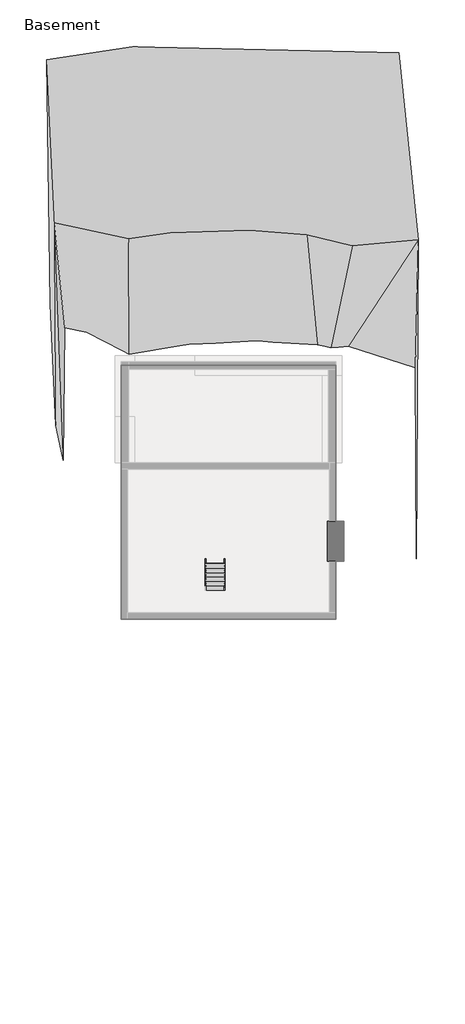
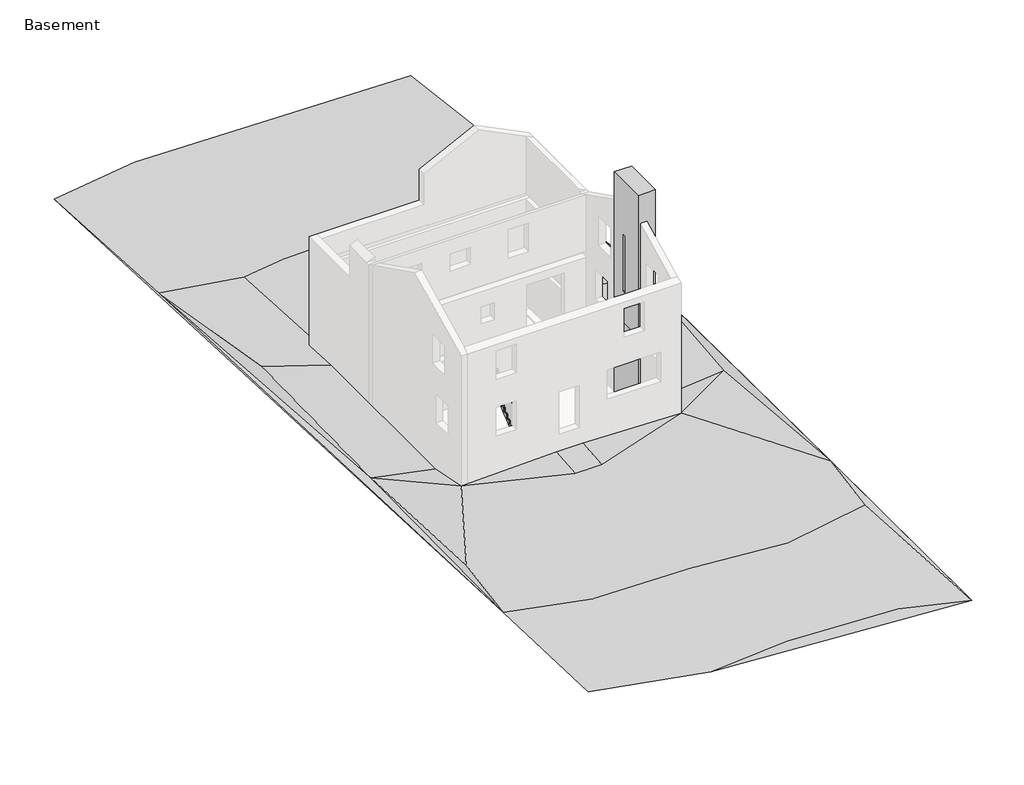
# One storey, part 2 of 2: 4 proxies, 2 members, 1 railing, 1 stair flight.
"""IFC4 building model written with IfcOpenShell, lengths in millimetres."""

import ifcopenshell
import ifcopenshell.guid

model = None  # the IFC model being written
_history = None  # IfcOwnerHistory: only IFC2X3 demands one
_inside = {}  # id of a spatial element -> (the spatial element, [elements in it])
_under = {}  # id of a project, library or spatial element -> (it, [spatial elements below it])
_declared = {}  # id of a project -> (the project, [libraries it declares])
_typed = {}  # id of a type object -> (the type object, [elements of that type])
_made_of = {}  # id of a material, layer set ... -> (it, [elements and type objects made of it])


def new_model(schema):
    """Start an empty IFC model of exactly this schema.

    Asked for "IFC4X3", IfcOpenShell would pick the latest addendum, in which some entities
    have other attributes; the version numbers below select the first issue.
    IFC2X3 requires an IfcOwnerHistory on every rooted entity: one is made here for all.
    """
    global model, _history
    if schema == "IFC4X3":
        model = ifcopenshell.file(schema_version=(4, 3, 0, 0))
    else:
        model = ifcopenshell.file(schema=schema)
    _inside.clear()
    _under.clear()
    _declared.clear()
    _typed.clear()
    _made_of.clear()
    _history = None
    if model.schema == "IFC2X3":
        org = make("IfcOrganization", Name="unknown")
        user = make(
            "IfcPersonAndOrganization",
            ThePerson=make("IfcPerson", FamilyName="unknown"),
            TheOrganization=org,
        )
        app = make(
            "IfcApplication",
            ApplicationDeveloper=org,
            Version="unknown",
            ApplicationFullName="unknown",
            ApplicationIdentifier="unknown",
        )
        _history = make(
            "IfcOwnerHistory",
            OwningUser=user,
            OwningApplication=app,
            ChangeAction="ADDED",
            CreationDate=0,
        )
    return model


def make(cls, **values):
    """One entity of the class cls with the attributes given. An attribute that is None is left unset."""
    return model.create_entity(
        cls, **{name: value for name, value in values.items() if value is not None}
    )


def rooted(cls, **values):
    """An entity with a GlobalId (a new one), such as an element, a storey or a relation."""
    return make(cls, GlobalId=ifcopenshell.guid.new(), OwnerHistory=_history, **values)


def si_unit(unit_type, name, prefix=None):
    """IfcSIUnit, for example si_unit("LENGTHUNIT", "METRE", prefix="MILLI")."""
    return make("IfcSIUnit", UnitType=unit_type, Prefix=prefix, Name=name)


def assignment(units):
    """IfcUnitAssignment: the units of a project."""
    return None if units is None else make("IfcUnitAssignment", Units=units)


def point(xyz):
    """IfcCartesianPoint."""
    return None if xyz is None else make("IfcCartesianPoint", Coordinates=xyz)


def direction(xyz):
    """IfcDirection."""
    return None if xyz is None else make("IfcDirection", DirectionRatios=xyz)


def frame(location, z_axis=None, x_axis=None):
    """IfcAxis2Placement3D, a coordinate frame: its origin and axes. An axis left out is left unset."""
    return make(
        "IfcAxis2Placement3D",
        Location=point(location),
        Axis=direction(z_axis),
        RefDirection=direction(x_axis),
    )


def origin():
    """The frame at (0, 0, 0) with its axes left unset."""
    return frame((0.0, 0.0, 0.0))


def place(relative_to, where):
    """IfcLocalPlacement: puts the frame where relative to a parent placement (None: the world)."""
    return make(
        "IfcLocalPlacement", PlacementRelTo=relative_to, RelativePlacement=where
    )


def context(
    kind, dimensions, precision=None, world=None, true_north=None, identifier=None
):
    """IfcGeometricRepresentationContext, for example the 3D "Model" context."""
    return make(
        "IfcGeometricRepresentationContext",
        ContextIdentifier=identifier,
        ContextType=kind,
        CoordinateSpaceDimension=dimensions,
        Precision=precision,
        WorldCoordinateSystem=world,
        TrueNorth=true_north,
    )


def project(units=None, contexts=None):
    """IfcProject with its units and contexts."""
    return rooted(
        "IfcProject",
        Name="project",
        RepresentationContexts=contexts,
        UnitsInContext=assignment(units),
    )


def spatial(cls, under=None, at=None, **own):
    """A site, building, storey or space (cls), placed at a placement, below another one or the project."""
    s = rooted(cls, ObjectPlacement=at, **own)
    if under is not None:
        _under.setdefault(under.id(), (under, []))[1].append(s)
    return s


def polyline(points):
    """IfcPolyline through the points."""
    return make("IfcPolyline", Points=[point(p) for p in points])


def point_list(points):
    """IfcCartesianPointList2D or 3D."""
    cls = (
        "IfcCartesianPointList2D" if len(points[0]) == 2 else "IfcCartesianPointList3D"
    )
    return make(cls, CoordList=points)


def outline(outer, holes=None, kind="AREA"):
    """IfcArbitraryClosedProfileDef: a profile drawn as a closed curve; with holes, ...WithVoids."""
    if holes is None:
        return make("IfcArbitraryClosedProfileDef", ProfileType=kind, OuterCurve=outer)
    return make(
        "IfcArbitraryProfileDefWithVoids",
        ProfileType=kind,
        OuterCurve=outer,
        InnerCurves=holes,
    )


def extrude(swept, where, along, depth):
    """IfcExtrudedAreaSolid: the profile swept, set in the frame where, extruded along a direction by depth."""
    return make(
        "IfcExtrudedAreaSolid",
        SweptArea=swept,
        Position=where,
        ExtrudedDirection=direction(along),
        Depth=depth,
    )


def faces_of(points, faces, orient=None, outer=None):
    """IfcFace entities. A face is a list of loops; a loop is a list of indices into points, from 0.

    orient and outer hold one flag for each loop. By default every Orientation is true, the
    first loop of a face is its IfcFaceOuterBound and the others are IfcFaceBound.
    """
    made = []
    for i, loops in enumerate(faces):
        bounds = []
        for j, loop in enumerate(loops):
            is_outer = j == 0 if outer is None else outer[i][j]
            bounds.append(
                make(
                    "IfcFaceOuterBound" if is_outer else "IfcFaceBound",
                    Bound=make("IfcPolyLoop", Polygon=[points[k] for k in loop]),
                    Orientation=True if orient is None else orient[i][j],
                )
            )
        made.append(make("IfcFace", Bounds=bounds))
    return made


def faceted_brep(points, faces, orient=None, outer=None, voids=None):
    """IfcFacetedBrep: a solid bounded by flat faces; with voids (closed shells), ...WithVoids."""
    shared = [point(p) for p in points]
    hull = make("IfcClosedShell", CfsFaces=faces_of(shared, faces, orient, outer))
    if voids is None:
        return make("IfcFacetedBrep", Outer=hull)
    return make(
        "IfcFacetedBrepWithVoids",
        Outer=hull,
        Voids=[
            make(cls, CfsFaces=faces_of(shared, fs, o, b)) for cls, fs, o, b in voids
        ],
    )


def triangles(points, corners, closed=None, point_numbers=None):
    """IfcTriangulatedFaceSet: each triangle names its three corners, points numbered from 1."""
    return make(
        "IfcTriangulatedFaceSet",
        Coordinates=point_list(points),
        Closed=closed,
        CoordIndex=corners,
        PnIndex=point_numbers,
    )


def shape(context_of_items, identifier, shape_type, items):
    """IfcShapeRepresentation: the items that make up one representation, for example the "Body"."""
    return make(
        "IfcShapeRepresentation",
        ContextOfItems=context_of_items,
        RepresentationIdentifier=identifier,
        RepresentationType=shape_type,
        Items=items,
    )


def source(mapping_origin, context_of_items, identifier, shape_type, items):
    """IfcRepresentationMap: a shape defined once, which mapped items show again and again."""
    return make(
        "IfcRepresentationMap",
        MappingOrigin=mapping_origin,
        MappedRepresentation=shape(context_of_items, identifier, shape_type, items),
    )


def transform(
    local_origin,
    x_axis=None,
    y_axis=None,
    z_axis=None,
    scale=None,
    scale2=None,
    scale3=None,
    uniform=True,
):
    """IfcCartesianTransformationOperator3D, or its non-uniform kind. x_axis, y_axis, z_axis: its Axis1, 2, 3."""
    if uniform:
        return make(
            "IfcCartesianTransformationOperator3D",
            Axis1=direction(x_axis),
            Axis2=direction(y_axis),
            LocalOrigin=point(local_origin),
            Scale=scale,
            Axis3=direction(z_axis),
        )
    return make(
        "IfcCartesianTransformationOperator3DnonUniform",
        Axis1=direction(x_axis),
        Axis2=direction(y_axis),
        LocalOrigin=point(local_origin),
        Scale=scale,
        Axis3=direction(z_axis),
        Scale2=scale2,
        Scale3=scale3,
    )


def mapped(mapping_source, mapping_target):
    """IfcMappedItem: shows the shape of a source again, moved by a transform."""
    return make(
        "IfcMappedItem", MappingSource=mapping_source, MappingTarget=mapping_target
    )


def made_of(thing, what):
    """Note that an element or type object is made of a material, layer set ...; save() writes the relation."""
    if what is not None:
        _made_of.setdefault(what.id(), (what, []))[1].append(thing)
    return thing


def element(
    cls,
    number,
    at=None,
    inside=None,
    cuts=None,
    type_object=None,
    material=None,
    context=None,
    identifier="Body",
    shape_type=None,
    held_by="IfcProductDefinitionShape",
    body=None,
    shapes=None,
    **own,
):
    """One element of the class cls, such as IfcWall. Its Tag is "e" and its number.

    at: its placement. inside: the storey or other place that contains it. cuts: it is an
    opening in that element (IfcRelVoidsElement). A single representation is given by context,
    identifier, shape_type and body (its items); several are given by shapes. held_by: the class
    of the entity that holds the representations. save() writes the other relations.
    """
    e = rooted(cls, Tag="e%d" % number, ObjectPlacement=at, **own)
    if body is not None:
        shapes = [shape(context, identifier, shape_type, body)]
    if shapes is not None:
        e.Representation = make(held_by, Representations=shapes)
    if inside is not None:
        _inside.setdefault(inside.id(), (inside, []))[1].append(e)
    if cuts is not None:
        rooted(
            "IfcRelVoidsElement", RelatingBuildingElement=cuts, RelatedOpeningElement=e
        )
    if type_object is not None:
        _typed.setdefault(type_object.id(), (type_object, []))[1].append(e)
    return made_of(e, material)


def aggregate(whole, parts):
    """IfcRelAggregates: a whole, such as a stair, and the parts it consists of."""
    return rooted("IfcRelAggregates", RelatingObject=whole, RelatedObjects=parts)


def save(model, path):
    """Write the relations noted so far, then the file.

    IfcRelAggregates (storeys below a building ...), IfcRelContainedInSpatialStructure (elements
    in a storey), IfcRelDefinesByType, IfcRelAssociatesMaterial and IfcRelDeclares: one each for
    every whole, place, type object, material and project.
    """
    for whole, parts in _under.values():
        aggregate(whole, parts)
    for where, things in _inside.values():
        rooted(
            "IfcRelContainedInSpatialStructure",
            RelatedElements=things,
            RelatingStructure=where,
        )
    for kind, things in _typed.values():
        rooted("IfcRelDefinesByType", RelatedObjects=things, RelatingType=kind)
    for what, things in _made_of.values():
        rooted("IfcRelAssociatesMaterial", RelatedObjects=things, RelatingMaterial=what)
    for by, libraries in _declared.values():
        rooted("IfcRelDeclares", RelatingContext=by, RelatedDefinitions=libraries)
    model.write(path)


def existing_fireplace_existing_fireplace_287aed51(model_context):
    return source(origin(), model_context, "Body", "Brep", [
        faceted_brep([(4450.2196932, 434.2888758, 8077.2), (3662.8196932, 434.2888758, 8077.2), (3662.8196932, -1445.3111242, 8077.2), (4450.2196932, -1445.3111242, 8077.2), (4450.2196932, 434.2888758, -2667.0), (4450.2196932, -1445.3111242, -2667.0), (4069.2196932, -1445.3111242, -2667.0), (3764.4196932, -1445.3111242, -2667.0), (3662.8196932, -1445.3111242, -2667.0), (3662.8196932, 434.2888758, -2667.0), (3764.4196932, 434.2888758, -2667.0), (4069.2196932, 434.2888758, -2667.0), (3662.8196932, 154.8888758, 0.0), (3662.8196932, 154.8888758, 1219.2), (3662.8196932, -1165.9111242, 1219.2), (3662.8196932, -1165.9111242, 0.0), (3662.8196932, -403.9111242, 5486.4), (3662.8196932, -403.9111242, 2743.2), (3662.8196932, -276.9111242, 2743.2), (3662.8196932, -276.9111242, 5486.4), (4145.4196932, -20.7631592, 1219.2), (4145.4196932, -990.2590891, 1219.2), (4145.4196932, -990.2590891, 0.0), (4145.4196932, -20.7631592, 0.0), (3767.2567114, -403.9111242, 5486.4), (3767.2567114, -403.9111242, 2743.2), (3767.2567114, -276.9111242, 2743.2), (3767.2567114, -276.9111242, 5486.4)], [[[0, 1, 2, 3]], [[4, 5, 6, 7, 8, 9, 10, 11]], [[1, 0, 4, 11, 10, 9]], [[2, 1, 9, 8], [12, 13, 14, 15], [16, 17, 18, 19]], [[3, 2, 8, 7, 6, 5]], [[0, 3, 5, 4]], [[14, 13, 20, 21]], [[15, 14, 21, 22]], [[21, 20, 23, 22]], [[13, 12, 23, 20]], [[12, 15, 22, 23]], [[24, 25, 17, 16]], [[26, 27, 19, 18]], [[25, 26, 18, 17]], [[25, 24, 27, 26]], [[27, 24, 16, 19]]]),
    ])


def stair_flight_b746b64e(model_context):
    return source(origin(), model_context, "Body", "SweptSolid", [
        extrude(outline(polyline([(-2791.5111242, -2476.5), (-2562.9111242, -2476.5), (-2562.9111242, -2527.3), (-2766.1111242, -2527.3), (-2766.1111242, -2520.95), (-2791.5111242, -2495.55), (-2791.5111242, -2476.5)])), frame((-2052.1803068, 0.0, 0.0), z_axis=(1.0, 0.0, 0.0), x_axis=(0.0, 1.0, 0.0)), (0.0, 0.0, 1.0), 939.8),
        extrude(outline(polyline([(-1112.3803068, -2759.7611242), (-1112.3803068, -2766.1111242), (-2052.1803068, -2766.1111242), (-2052.1803068, -2759.7611242), (-1112.3803068, -2759.7611242)])), frame((0.0, 0.0, -2667.0), z_axis=(0.0, 0.0, 1.0), x_axis=(1.0, 0.0, 0.0)), (0.0, 0.0, 1.0), 139.7),
        extrude(outline(polyline([(-1112.3803068, -2556.5611242), (-1112.3803068, -2562.9111242), (-2052.1803068, -2562.9111242), (-2052.1803068, -2556.5611242), (-1112.3803068, -2556.5611242)])), frame((0.0, 0.0, -2527.3), z_axis=(0.0, 0.0, 1.0), x_axis=(1.0, 0.0, 0.0)), (0.0, 0.0, 1.0), 190.5),
        extrude(outline(polyline([(-2588.3111242, -2286.0), (-2359.7111242, -2286.0), (-2359.7111242, -2336.8), (-2562.9111242, -2336.8), (-2562.9111242, -2330.45), (-2588.3111242, -2305.05), (-2588.3111242, -2286.0)])), frame((-2052.1803068, 0.0, 0.0), z_axis=(1.0, 0.0, 0.0), x_axis=(0.0, 1.0, 0.0)), (0.0, 0.0, 1.0), 939.8),
        extrude(outline(polyline([(-1112.3803068, -2353.3611242), (-1112.3803068, -2359.7111242), (-2052.1803068, -2359.7111242), (-2052.1803068, -2353.3611242), (-1112.3803068, -2353.3611242)])), frame((0.0, 0.0, -2336.8), z_axis=(0.0, 0.0, 1.0), x_axis=(1.0, 0.0, 0.0)), (0.0, 0.0, 1.0), 190.5),
        extrude(outline(polyline([(-2385.1111242, -2095.5), (-2156.5111242, -2095.5), (-2156.5111242, -2146.3), (-2359.7111242, -2146.3), (-2359.7111242, -2139.95), (-2385.1111242, -2114.55), (-2385.1111242, -2095.5)])), frame((-2052.1803068, 0.0, 0.0), z_axis=(1.0, 0.0, 0.0), x_axis=(0.0, 1.0, 0.0)), (0.0, 0.0, 1.0), 939.8),
        extrude(outline(polyline([(-1112.3803068, -2150.1611242), (-1112.3803068, -2156.5111242), (-2052.1803068, -2156.5111242), (-2052.1803068, -2150.1611242), (-1112.3803068, -2150.1611242)])), frame((0.0, 0.0, -2146.3), z_axis=(0.0, 0.0, 1.0), x_axis=(1.0, 0.0, 0.0)), (0.0, 0.0, 1.0), 190.5),
        extrude(outline(polyline([(-2181.9111242, -1905.0), (-1953.3111242, -1905.0), (-1953.3111242, -1955.8), (-2156.5111242, -1955.8), (-2156.5111242, -1949.45), (-2181.9111242, -1924.05), (-2181.9111242, -1905.0)])), frame((-2052.1803068, 0.0, 0.0), z_axis=(1.0, 0.0, 0.0), x_axis=(0.0, 1.0, 0.0)), (0.0, 0.0, 1.0), 939.8),
        extrude(outline(polyline([(-1112.3803068, -1946.9611242), (-1112.3803068, -1953.3111242), (-2052.1803068, -1953.3111242), (-2052.1803068, -1946.9611242), (-1112.3803068, -1946.9611242)])), frame((0.0, 0.0, -1955.8), z_axis=(0.0, 0.0, 1.0), x_axis=(1.0, 0.0, 0.0)), (0.0, 0.0, 1.0), 190.5),
        extrude(outline(polyline([(-1978.7111242, -1714.5), (-1750.1111242, -1714.5), (-1750.1111242, -1765.3), (-1953.3111242, -1765.3), (-1953.3111242, -1758.95), (-1978.7111242, -1733.55), (-1978.7111242, -1714.5)])), frame((-2052.1803068, 0.0, 0.0), z_axis=(1.0, 0.0, 0.0), x_axis=(0.0, 1.0, 0.0)), (0.0, 0.0, 1.0), 939.8),
        extrude(outline(polyline([(-1112.3803068, -1743.7611242), (-1112.3803068, -1750.1111242), (-2052.1803068, -1750.1111242), (-2052.1803068, -1743.7611242), (-1112.3803068, -1743.7611242)])), frame((0.0, 0.0, -1765.3), z_axis=(0.0, 0.0, 1.0), x_axis=(1.0, 0.0, 0.0)), (0.0, 0.0, 1.0), 190.5),
        extrude(outline(polyline([(-1775.5111242, -1524.0), (-1546.9111242, -1524.0), (-1546.9111242, -1574.8), (-1750.1111242, -1574.8), (-1750.1111242, -1568.45), (-1775.5111242, -1543.05), (-1775.5111242, -1524.0)])), frame((-2052.1803068, 0.0, 0.0), z_axis=(1.0, 0.0, 0.0), x_axis=(0.0, 1.0, 0.0)), (0.0, 0.0, 1.0), 939.8),
        extrude(outline(polyline([(-1112.3803068, -1540.5611242), (-1112.3803068, -1546.9111242), (-2052.1803068, -1546.9111242), (-2052.1803068, -1540.5611242), (-1112.3803068, -1540.5611242)])), frame((0.0, 0.0, -1574.8), z_axis=(0.0, 0.0, 1.0), x_axis=(1.0, 0.0, 0.0)), (0.0, 0.0, 1.0), 190.5),
        extrude(outline(polyline([(-1572.3111242, -1333.5), (-1343.7111242, -1333.5), (-1343.7111242, -1384.3), (-1546.9111242, -1384.3), (-1546.9111242, -1377.95), (-1572.3111242, -1352.55), (-1572.3111242, -1333.5)])), frame((-2052.1803068, 0.0, 0.0), z_axis=(1.0, 0.0, 0.0), x_axis=(0.0, 1.0, 0.0)), (0.0, 0.0, 1.0), 939.8),
        extrude(outline(polyline([(-1112.3803068, -1337.3611242), (-1112.3803068, -1343.7111242), (-2052.1803068, -1343.7111242), (-2052.1803068, -1337.3611242), (-1112.3803068, -1337.3611242)])), frame((0.0, 0.0, -1384.3), z_axis=(0.0, 0.0, 1.0), x_axis=(1.0, 0.0, 0.0)), (0.0, 0.0, 1.0), 190.5),
        extrude(outline(polyline([(-1369.1111242, -1143.0), (-1140.5111242, -1143.0), (-1140.5111242, -1193.8), (-1343.7111242, -1193.8), (-1343.7111242, -1187.45), (-1369.1111242, -1162.05), (-1369.1111242, -1143.0)])), frame((-2052.1803068, 0.0, 0.0), z_axis=(1.0, 0.0, 0.0), x_axis=(0.0, 1.0, 0.0)), (0.0, 0.0, 1.0), 939.8),
        extrude(outline(polyline([(-1112.3803068, -1134.1611242), (-1112.3803068, -1140.5111242), (-2052.1803068, -1140.5111242), (-2052.1803068, -1134.1611242), (-1112.3803068, -1134.1611242)])), frame((0.0, 0.0, -1193.8), z_axis=(0.0, 0.0, 1.0), x_axis=(1.0, 0.0, 0.0)), (0.0, 0.0, 1.0), 190.5),
        extrude(outline(polyline([(-1165.9111242, -952.5), (-937.3111242, -952.5), (-937.3111242, -1003.3), (-1140.5111242, -1003.3), (-1140.5111242, -996.95), (-1165.9111242, -971.55), (-1165.9111242, -952.5)])), frame((-2052.1803068, 0.0, 0.0), z_axis=(1.0, 0.0, 0.0), x_axis=(0.0, 1.0, 0.0)), (0.0, 0.0, 1.0), 939.8),
        extrude(outline(polyline([(-1112.3803068, -930.9611242), (-1112.3803068, -937.3111242), (-2052.1803068, -937.3111242), (-2052.1803068, -930.9611242), (-1112.3803068, -930.9611242)])), frame((0.0, 0.0, -1003.3), z_axis=(0.0, 0.0, 1.0), x_axis=(1.0, 0.0, 0.0)), (0.0, 0.0, 1.0), 190.5),
        extrude(outline(polyline([(-962.7111242, -762.0), (-734.1111242, -762.0), (-734.1111242, -812.8), (-937.3111242, -812.8), (-937.3111242, -806.45), (-962.7111242, -781.05), (-962.7111242, -762.0)])), frame((-2052.1803068, 0.0, 0.0), z_axis=(1.0, 0.0, 0.0), x_axis=(0.0, 1.0, 0.0)), (0.0, 0.0, 1.0), 939.8),
        extrude(outline(polyline([(-1112.3803068, -727.7611242), (-1112.3803068, -734.1111242), (-2052.1803068, -734.1111242), (-2052.1803068, -727.7611242), (-1112.3803068, -727.7611242)])), frame((0.0, 0.0, -812.8), z_axis=(0.0, 0.0, 1.0), x_axis=(1.0, 0.0, 0.0)), (0.0, 0.0, 1.0), 190.5),
        extrude(outline(polyline([(-759.5111242, -571.5), (-530.9111242, -571.5), (-530.9111242, -622.3), (-734.1111242, -622.3), (-734.1111242, -615.95), (-759.5111242, -590.55), (-759.5111242, -571.5)])), frame((-2052.1803068, 0.0, 0.0), z_axis=(1.0, 0.0, 0.0), x_axis=(0.0, 1.0, 0.0)), (0.0, 0.0, 1.0), 939.8),
        extrude(outline(polyline([(-1112.3803068, -524.5611242), (-1112.3803068, -530.9111242), (-2052.1803068, -530.9111242), (-2052.1803068, -524.5611242), (-1112.3803068, -524.5611242)])), frame((0.0, 0.0, -622.3), z_axis=(0.0, 0.0, 1.0), x_axis=(1.0, 0.0, 0.0)), (0.0, 0.0, 1.0), 190.5),
        extrude(outline(polyline([(-556.3111242, -381.0), (-327.7111242, -381.0), (-327.7111242, -431.8), (-530.9111242, -431.8), (-530.9111242, -425.45), (-556.3111242, -400.05), (-556.3111242, -381.0)])), frame((-2052.1803068, 0.0, 0.0), z_axis=(1.0, 0.0, 0.0), x_axis=(0.0, 1.0, 0.0)), (0.0, 0.0, 1.0), 939.8),
        extrude(outline(polyline([(-1112.3803068, -321.3611242), (-1112.3803068, -327.7111242), (-2052.1803068, -327.7111242), (-2052.1803068, -321.3611242), (-1112.3803068, -321.3611242)])), frame((0.0, 0.0, -431.8), z_axis=(0.0, 0.0, 1.0), x_axis=(1.0, 0.0, 0.0)), (0.0, 0.0, 1.0), 190.5),
        extrude(outline(polyline([(-353.1111242, -190.5), (-124.5111242, -190.5), (-124.5111242, -241.3), (-327.7111242, -241.3), (-327.7111242, -234.95), (-353.1111242, -209.55), (-353.1111242, -190.5)])), frame((-2052.1803068, 0.0, 0.0), z_axis=(1.0, 0.0, 0.0), x_axis=(0.0, 1.0, 0.0)), (0.0, 0.0, 1.0), 939.8),
        extrude(outline(polyline([(-1112.3803068, -118.1611242), (-1112.3803068, -124.5111242), (-2052.1803068, -124.5111242), (-2052.1803068, -118.1611242), (-1112.3803068, -118.1611242)])), frame((0.0, 0.0, -241.3), z_axis=(0.0, 0.0, 1.0), x_axis=(1.0, 0.0, 0.0)), (0.0, 0.0, 1.0), 190.5),
    ])


model = new_model("IFC4")

# Units and contexts
model_context = context("Model", 3, world=origin())
ifc_project = project(units=[si_unit("LENGTHUNIT", "METRE", prefix="MILLI")], contexts=[model_context])

# Site, building, storey
site = spatial("IfcSite", under=ifc_project)
building = spatial("IfcBuilding", under=site)
storey = spatial("IfcBuildingStorey", under=building, Name="Basement", Elevation=-2667.0)

# Proxies
placement = place(None, origin())
element("IfcBuildingElementProxy", 1, Name="Building Element Proxy", at=placement, inside=storey, context=model_context, shape_type="Tessellation", body=[
    triangles([(-9474.14729, 22003.2871765, -1727.1999516), (-8916.1412338, -12566.1132111, -939.7999758), (-8632.7724838, -18803.3999359, -1092.1999758), (-3754.3850807, -20036.8885986, -1092.1999758), (7677.2023224, -20906.8378235, -1092.1999758), (7936.7585724, 13587.9496765, -1752.6), (7012.0400162, 22339.8364014, -1727.1999516), (-5437.1349838, 22620.8239014, -1727.1999516), (4069.2196426, 434.2888621, -1346.1999516), (4450.2196426, 434.2888621, -1346.1999516), (4450.2196426, -349.5066825, -1346.1999516), (4450.2196426, -1445.3110531, -1346.1999516), (4069.2196426, -1445.3110531, -1346.1999516), (4069.2196426, -2313.9084709, -1346.1999516), (4069.2196426, -4163.1110046, -939.7999758), (-426.580321, -4163.1110046, -812.8000242), (-1645.7803574, -4163.1110046, -812.8000242), (-5989.1803574, -4163.1110046, -939.7999758), (-5989.1803574, -2124.4043404, -1346.1999516), (-5989.1803574, 3152.0889954, -1346.1999516), (-5989.1803574, 4989.0600082, -1346.1999516), (-5989.1803574, 6156.3282944, -1346.1999516), (-5989.1803574, 7724.0889954, -1429.2445919), (-5611.7969971, 7724.0889954, -1439.6358181), (-2815.8938187, 7724.0889954, -1415.0254017), (-2474.4123367, 7724.0889954, -1412.4145145), (-1876.9665367, 7724.0889954, -1411.4359406), (391.3462071, 7724.0889954, -1403.6252254), (781.867392, 7724.0889954, -1405.4288944), (3306.7437996, 7724.0889954, -1413.4377079), (3676.8014442, 7724.0889954, -1418.4369667), (4069.2196426, 7724.0889954, -1416.2554138), (4069.2196426, 7529.9159637, -1404.4058464), (4069.2196426, 6299.0253983, -1346.1999516), (4069.2196426, 3152.0889954, -1346.1999516), (-9109.81604, 14372.1750641, -1752.6), (-8549.4287338, -9013.2876297, -939.7999758), (-8523.2349838, -1401.2252266, -1346.1999516), (-8408.9349838, 7414.1625641, -1346.1999516), (-6082.4537338, -10022.9382111, -939.7999758), (-5633.19104, 13643.5125641, -1752.6), (-5382.3662338, -13518.6132111, -939.7999758), (-3671.0413307, 13924.5000641, -1752.6), (-2942.3788307, -9965.7882111, -939.7999758), (-1568.3975807, 21947.7254517, -1727.1999516), (-840.5287823, -13629.7378235, -939.7999758), (-699.241258, -10470.6132111, -939.7999758), (-109.4850414, -19700.3370483, -1092.1999758), (29.4212079, 14035.6246765, -1752.6), (2721.8210724, 13811.7871765, -1752.6), (2805.1648224, 21892.1614014, -1727.1999516), (3252.0462662, -14021.8499359, -939.7999758), (4179.1460724, -9854.6624359, -939.7999758), (4845.1025162, -19962.2745483, -1092.1999758), (4852.2462662, 13306.9621765, -1752.6), (7177.93396, -13294.7757111, -939.7999758), (7289.85271, -1961.6126781, -1346.1999516), (7543.0587662, -9965.7882111, -939.7999758), (7740.7025162, 5059.8998703, -1346.1999516), (-1645.7803574, -5668.0610046, -939.7999758), (-426.580321, -5668.0610046, -939.7999758)], [[40, 2, 42], [42, 2, 3], [2, 40, 37], [37, 38, 2], [38, 37, 18], [18, 19, 38], [37, 40, 18], [38, 19, 20], [40, 60, 18], [2, 38, 36], [42, 4, 46], [4, 42, 3], [42, 46, 44], [47, 46, 52], [4, 48, 46], [44, 46, 47], [60, 17, 18], [44, 47, 60], [61, 16, 17], [17, 60, 61], [40, 44, 60], [60, 47, 61], [44, 40, 42], [21, 22, 39], [20, 21, 39], [8, 1, 36], [36, 1, 2], [36, 39, 41], [23, 39, 22], [36, 38, 39], [23, 41, 39], [20, 39, 38], [41, 24, 25], [25, 26, 43], [27, 43, 26], [41, 8, 36], [8, 41, 43], [43, 45, 8], [49, 45, 43], [41, 25, 43], [8, 45, 51], [49, 43, 27], [24, 41, 23], [52, 53, 47], [52, 48, 54], [53, 52, 56], [47, 53, 61], [14, 15, 57], [61, 53, 15], [13, 14, 12], [58, 15, 53], [52, 46, 48], [56, 58, 53], [56, 54, 5], [58, 5, 59], [5, 58, 56], [54, 48, 5], [58, 57, 15], [10, 11, 57], [12, 57, 11], [12, 14, 57], [10, 57, 59], [58, 59, 57], [56, 52, 54], [48, 4, 5], [49, 28, 29], [50, 29, 30], [49, 50, 51], [49, 29, 50], [31, 55, 30], [50, 55, 51], [50, 30, 55], [49, 51, 45], [49, 27, 28], [34, 35, 59], [33, 59, 32], [59, 33, 34], [9, 10, 35], [32, 55, 31], [55, 32, 6], [6, 7, 55], [32, 59, 6], [55, 7, 51], [59, 5, 6], [10, 59, 35], [51, 7, 8], [16, 61, 15]], closed=False),
])
element("IfcBuildingElementProxy", 2, Name="Building Element Proxy", at=placement, inside=storey, context=model_context, shape_type="Tessellation", body=[
    triangles([(4069.2196426, 3152.0889954, -3073.5594864), (4069.2196426, 3152.0889954, -1346.1999516), (4069.2196426, 434.2888621, -3073.5594864), (4069.2196426, 434.2888621, -1346.1999516), (4450.2196426, 434.2888621, -3073.5594864), (4450.2196426, 434.2888621, -1346.1999516), (4450.2196426, -349.5066825, -3073.5594864), (4450.2196426, -349.5066825, -1346.1999516), (4450.2196426, -1445.3110531, -3073.5594864), (4450.2196426, -1445.3110531, -1346.1999516), (4069.2196426, -1445.3110531, -3073.5594864), (4069.2196426, -1445.3110531, -1346.1999516), (4069.2196426, -2313.9084709, -3073.5594864), (4069.2196426, -2313.9084709, -1346.1999516), (4069.2196426, -4163.1110046, -3073.5594864), (4069.2196426, -4163.1110046, -939.7999758), (-426.580321, -4163.1110046, -3073.5594864), (-426.580321, -4163.1110046, -812.8000242), (-1645.7803574, -4163.1110046, -3073.5594864), (-1645.7803574, -4163.1110046, -812.8000242), (-5989.1803574, -4163.1110046, -3073.5594864), (-5989.1803574, -4163.1110046, -939.7999758), (-5989.1803574, -2124.4043404, -3073.5594864), (-5989.1803574, -2124.4043404, -1346.1999516), (-5989.1803574, 3152.0889954, -3073.5594864), (-5989.1803574, 3152.0889954, -1346.1999516)], [[1, 4, 2], [1, 3, 4], [3, 6, 4], [3, 5, 6], [5, 8, 6], [5, 7, 8], [7, 10, 8], [7, 9, 10], [9, 12, 10], [9, 11, 12], [11, 14, 12], [11, 13, 14], [13, 16, 14], [13, 15, 16], [15, 18, 16], [15, 17, 18], [17, 20, 18], [17, 19, 20], [19, 22, 20], [19, 21, 22], [21, 24, 22], [21, 23, 24], [23, 26, 24], [23, 25, 26]], closed=False),
    triangles([(4069.2196426, 434.2888621, -3073.5594864), (4069.2196426, 3152.0889954, -3073.5594864), (-5989.1803574, 3152.0889954, -3073.5594864), (-5989.1803574, -4163.1110046, -3073.5594864), (4069.2196426, -4163.1110046, -3073.5594864), (4069.2196426, -1445.3110531, -3073.5594864), (4450.2196426, -1445.3110531, -3073.5594864), (4450.2196426, 434.2888621, -3073.5594864)], [[4, 6, 3], [6, 4, 5], [3, 1, 2], [1, 3, 6], [6, 7, 1], [8, 1, 7]], closed=False),
])
element("IfcBuildingElementProxy", 3, Name="Building Element Proxy", at=placement, inside=storey, context=model_context, shape_type="Tessellation", body=[
    triangles([(-5989.1803574, 3152.0889954, -3073.5594864), (-5989.1803574, 3152.0889954, -1346.1999516), (-5989.1803574, 4989.0600082, -3073.5594864), (-5989.1803574, 4989.0600082, -1346.1999516), (-5989.1803574, 6156.3282944, -3073.5594864), (-5989.1803574, 6156.3282944, -1346.1999516), (-5989.1803574, 7724.0889954, -3073.5594864), (-5989.1803574, 7724.0889954, -1429.2445919), (-5611.7969971, 7724.0889954, -3073.5594864), (-5611.7969971, 7724.0889954, -1439.6358181), (-2815.8938187, 7724.0889954, -3073.5594864), (-2815.8938187, 7724.0889954, -1415.0254017), (-2474.4123367, 7724.0889954, -3073.5594864), (-2474.4123367, 7724.0889954, -1412.4145145), (-1876.9665367, 7724.0889954, -3073.5594864), (-1876.9665367, 7724.0889954, -1411.4359406), (391.3462071, 7724.0889954, -3073.5594864), (391.3462071, 7724.0889954, -1403.6252254), (781.867392, 7724.0889954, -3073.5594864), (781.867392, 7724.0889954, -1405.4288944), (3306.7437996, 7724.0889954, -3073.5594864), (3306.7437996, 7724.0889954, -1413.4377079), (3676.8014442, 7724.0889954, -3073.5594864), (3676.8014442, 7724.0889954, -1418.4369667), (4069.2196426, 7724.0889954, -3073.5594864), (4069.2196426, 7724.0889954, -1416.2554138), (4069.2196426, 7529.9159637, -3073.5594864), (4069.2196426, 7529.9159637, -1404.4058464), (4069.2196426, 6299.0253983, -3073.5594864), (4069.2196426, 6299.0253983, -1346.1999516), (4069.2196426, 3152.0889954, -3073.5594864), (4069.2196426, 3152.0889954, -1346.1999516)], [[1, 4, 2], [1, 3, 4], [3, 6, 4], [3, 5, 6], [5, 8, 6], [5, 7, 8], [7, 10, 8], [7, 9, 10], [9, 12, 10], [9, 11, 12], [11, 14, 12], [11, 13, 14], [13, 16, 14], [13, 15, 16], [15, 18, 16], [15, 17, 18], [17, 20, 18], [17, 19, 20], [19, 22, 20], [19, 21, 22], [21, 24, 22], [21, 23, 24], [23, 26, 24], [23, 25, 26], [25, 28, 26], [25, 27, 28], [27, 30, 28], [27, 29, 30], [29, 32, 30], [29, 31, 32]], closed=False),
    triangles([(-5989.1803574, 7724.0889954, -3073.5594864), (-5989.1803574, 3152.0889954, -3073.5594864), (4069.2196426, 3152.0889954, -3073.5594864), (4069.2196426, 7724.0889954, -3073.5594864)], [[1, 2, 4], [3, 4, 2]], closed=False),
])
existing_fireplace_existing_fireplace_shape = existing_fireplace_existing_fireplace_287aed51(model_context)
element("IfcBuildingElementProxy", 4, Name="Existing Fireplace : Existing Fireplace", ObjectType="Existing Fireplace : Existing Fireplace", at=placement, inside=storey, context=model_context, shape_type="MappedRepresentation", body=[
    mapped(existing_fireplace_existing_fireplace_shape, transform((0.0, 0.0, 0.0), x_axis=(1.0, 0.0, 0.0), y_axis=(0.0, 1.0, 0.0), z_axis=(0.0, 0.0, 1.0))),
])

# Members
element("IfcMember", 5, at=placement, inside=storey, context=model_context, shape_type="Brep", body=[
    faceted_brep([(-2052.1803068, -2759.7611242, -2667.0), (-2052.1803068, -2612.7302092, -2667.0), (-2001.3803068, -2612.7302092, -2667.0), (-2001.3803068, -2759.7611242, -2667.0), (-2001.3803068, -149.9111242, -358.1071078), (-2052.1803068, -149.9111242, -358.1071078), (-2052.1803068, -149.9111242, -241.3), (-2001.3803068, -149.9111242, -241.3), (-2052.1803068, -2556.5611242, -2614.3414828), (-2052.1803068, -2353.3611242, -2423.8414828), (-2052.1803068, -2150.1611242, -2233.3414828), (-2052.1803068, -1946.9611242, -2042.8414828), (-2052.1803068, -1743.7611242, -1852.3414828), (-2052.1803068, -1540.5611242, -1661.8414828), (-2052.1803068, -1337.3611242, -1471.3414828), (-2052.1803068, -1134.1611242, -1280.8414828), (-2052.1803068, -930.9611242, -1090.3414828), (-2052.1803068, -727.7611242, -899.8414828), (-2052.1803068, -524.5611242, -709.3414828), (-2052.1803068, -321.3611242, -518.8414828), (-2052.1803068, -2759.7611242, -2527.3), (-2052.1803068, -2556.5611242, -2527.3), (-2052.1803068, -2556.5611242, -2336.8), (-2052.1803068, -2353.3611242, -2336.8), (-2052.1803068, -2353.3611242, -2146.3), (-2052.1803068, -2150.1611242, -2146.3), (-2052.1803068, -2150.1611242, -1955.8), (-2052.1803068, -1946.9611242, -1955.8), (-2052.1803068, -1946.9611242, -1765.3), (-2052.1803068, -1743.7611242, -1765.3), (-2052.1803068, -1743.7611242, -1574.8), (-2052.1803068, -1540.5611242, -1574.8), (-2052.1803068, -1540.5611242, -1384.3), (-2052.1803068, -1337.3611242, -1384.3), (-2052.1803068, -1337.3611242, -1193.8), (-2052.1803068, -1134.1611242, -1193.8), (-2052.1803068, -1134.1611242, -1003.3), (-2052.1803068, -930.9611242, -1003.3), (-2052.1803068, -930.9611242, -812.8), (-2052.1803068, -727.7611242, -812.8), (-2052.1803068, -727.7611242, -622.3), (-2052.1803068, -524.5611242, -622.3), (-2052.1803068, -524.5611242, -431.8), (-2052.1803068, -321.3611242, -431.8), (-2052.1803068, -321.3611242, -241.3), (-2001.3803068, -321.3611242, -241.3), (-2001.3803068, -321.3611242, -431.8), (-2001.3803068, -524.5611242, -431.8), (-2001.3803068, -524.5611242, -622.3), (-2001.3803068, -727.7611242, -622.3), (-2001.3803068, -727.7611242, -812.8), (-2001.3803068, -930.9611242, -812.8), (-2001.3803068, -930.9611242, -1003.3), (-2001.3803068, -1134.1611242, -1003.3), (-2001.3803068, -1134.1611242, -1193.8), (-2001.3803068, -1337.3611242, -1193.8), (-2001.3803068, -1337.3611242, -1384.3), (-2001.3803068, -1540.5611242, -1384.3), (-2001.3803068, -1540.5611242, -1574.8), (-2001.3803068, -1743.7611242, -1574.8), (-2001.3803068, -1743.7611242, -1765.3), (-2001.3803068, -1946.9611242, -1765.3), (-2001.3803068, -1946.9611242, -1955.8), (-2001.3803068, -2150.1611242, -1955.8), (-2001.3803068, -2150.1611242, -2146.3), (-2001.3803068, -2353.3611242, -2146.3), (-2001.3803068, -2353.3611242, -2336.8), (-2001.3803068, -2556.5611242, -2336.8), (-2001.3803068, -2556.5611242, -2527.3), (-2001.3803068, -2759.7611242, -2527.3)], [[[0, 1, 2, 3]], [[4, 5, 6, 7]], [[5, 4, 2, 1, 8, 9, 10, 11, 12, 13, 14, 15, 16, 17, 18, 19]], [[6, 5, 19, 18, 17, 16, 15, 14, 13, 12, 11, 10, 9, 8, 1, 0, 20, 21, 22, 23, 24, 25, 26, 27, 28, 29, 30, 31, 32, 33, 34, 35, 36, 37, 38, 39, 40, 41, 42, 43, 44]], [[44, 45, 7, 6]], [[4, 7, 45, 46, 47, 48, 49, 50, 51, 52, 53, 54, 55, 56, 57, 58, 59, 60, 61, 62, 63, 64, 65, 66, 67, 68, 69, 3, 2]], [[69, 20, 0, 3]], [[20, 69, 68, 21]], [[21, 68, 67, 22]], [[22, 67, 66, 23]], [[23, 66, 65, 24]], [[24, 65, 64, 25]], [[25, 64, 63, 26]], [[26, 63, 62, 27]], [[27, 62, 61, 28]], [[28, 61, 60, 29]], [[29, 60, 59, 30]], [[30, 59, 58, 31]], [[31, 58, 57, 32]], [[32, 57, 56, 33]], [[33, 56, 55, 34]], [[34, 55, 54, 35]], [[35, 54, 53, 36]], [[36, 53, 52, 37]], [[37, 52, 51, 38]], [[38, 51, 50, 39]], [[39, 50, 49, 40]], [[40, 49, 48, 41]], [[41, 48, 47, 42]], [[42, 47, 46, 43]], [[43, 46, 45, 44]]]),
])
element("IfcMember", 6, at=placement, inside=storey, context=model_context, shape_type="Brep", body=[
    faceted_brep([(-1163.1803068, -2759.7611242, -2667.0), (-1163.1803068, -2612.7302092, -2667.0), (-1112.3803068, -2612.7302092, -2667.0), (-1112.3803068, -2759.7611242, -2667.0), (-1112.3803068, -149.9111242, -358.1071078), (-1163.1803068, -149.9111242, -358.1071078), (-1163.1803068, -149.9111242, -241.3), (-1112.3803068, -149.9111242, -241.3), (-1112.3803068, -321.3611242, -518.8414828), (-1112.3803068, -524.5611242, -709.3414828), (-1112.3803068, -727.7611242, -899.8414828), (-1112.3803068, -930.9611242, -1090.3414828), (-1112.3803068, -1134.1611242, -1280.8414828), (-1112.3803068, -1337.3611242, -1471.3414828), (-1112.3803068, -1540.5611242, -1661.8414828), (-1112.3803068, -1743.7611242, -1852.3414828), (-1112.3803068, -1946.9611242, -2042.8414828), (-1112.3803068, -2150.1611242, -2233.3414828), (-1112.3803068, -2353.3611242, -2423.8414828), (-1112.3803068, -2556.5611242, -2614.3414828), (-1163.1803068, -2759.7611242, -2527.3), (-1163.1803068, -2556.5611242, -2527.3), (-1163.1803068, -2556.5611242, -2336.8), (-1163.1803068, -2353.3611242, -2336.8), (-1163.1803068, -2353.3611242, -2146.3), (-1163.1803068, -2150.1611242, -2146.3), (-1163.1803068, -2150.1611242, -1955.8), (-1163.1803068, -1946.9611242, -1955.8), (-1163.1803068, -1946.9611242, -1765.3), (-1163.1803068, -1743.7611242, -1765.3), (-1163.1803068, -1743.7611242, -1574.8), (-1163.1803068, -1540.5611242, -1574.8), (-1163.1803068, -1540.5611242, -1384.3), (-1163.1803068, -1337.3611242, -1384.3), (-1163.1803068, -1337.3611242, -1193.8), (-1163.1803068, -1134.1611242, -1193.8), (-1163.1803068, -1134.1611242, -1003.3), (-1163.1803068, -930.9611242, -1003.3), (-1163.1803068, -930.9611242, -812.8), (-1163.1803068, -727.7611242, -812.8), (-1163.1803068, -727.7611242, -622.3), (-1163.1803068, -524.5611242, -622.3), (-1163.1803068, -524.5611242, -431.8), (-1163.1803068, -321.3611242, -431.8), (-1163.1803068, -321.3611242, -241.3), (-1112.3803068, -321.3611242, -241.3), (-1112.3803068, -321.3611242, -431.8), (-1112.3803068, -524.5611242, -431.8), (-1112.3803068, -524.5611242, -622.3), (-1112.3803068, -727.7611242, -622.3), (-1112.3803068, -727.7611242, -812.8), (-1112.3803068, -930.9611242, -812.8), (-1112.3803068, -930.9611242, -1003.3), (-1112.3803068, -1134.1611242, -1003.3), (-1112.3803068, -1134.1611242, -1193.8), (-1112.3803068, -1337.3611242, -1193.8), (-1112.3803068, -1337.3611242, -1384.3), (-1112.3803068, -1540.5611242, -1384.3), (-1112.3803068, -1540.5611242, -1574.8), (-1112.3803068, -1743.7611242, -1574.8), (-1112.3803068, -1743.7611242, -1765.3), (-1112.3803068, -1946.9611242, -1765.3), (-1112.3803068, -1946.9611242, -1955.8), (-1112.3803068, -2150.1611242, -1955.8), (-1112.3803068, -2150.1611242, -2146.3), (-1112.3803068, -2353.3611242, -2146.3), (-1112.3803068, -2353.3611242, -2336.8), (-1112.3803068, -2556.5611242, -2336.8), (-1112.3803068, -2556.5611242, -2527.3), (-1112.3803068, -2759.7611242, -2527.3)], [[[0, 1, 2, 3]], [[4, 5, 6, 7]], [[5, 4, 8, 9, 10, 11, 12, 13, 14, 15, 16, 17, 18, 19, 2, 1]], [[6, 5, 1, 0, 20, 21, 22, 23, 24, 25, 26, 27, 28, 29, 30, 31, 32, 33, 34, 35, 36, 37, 38, 39, 40, 41, 42, 43, 44]], [[44, 45, 7, 6]], [[4, 7, 45, 46, 47, 48, 49, 50, 51, 52, 53, 54, 55, 56, 57, 58, 59, 60, 61, 62, 63, 64, 65, 66, 67, 68, 69, 3, 2, 19, 18, 17, 16, 15, 14, 13, 12, 11, 10, 9, 8]], [[69, 20, 0, 3]], [[20, 69, 68, 21]], [[21, 68, 67, 22]], [[22, 67, 66, 23]], [[23, 66, 65, 24]], [[24, 65, 64, 25]], [[25, 64, 63, 26]], [[26, 63, 62, 27]], [[27, 62, 61, 28]], [[28, 61, 60, 29]], [[29, 60, 59, 30]], [[30, 59, 58, 31]], [[31, 58, 57, 32]], [[32, 57, 56, 33]], [[33, 56, 55, 34]], [[34, 55, 54, 35]], [[35, 54, 53, 36]], [[36, 53, 52, 37]], [[37, 52, 51, 38]], [[38, 51, 50, 39]], [[39, 50, 49, 40]], [[40, 49, 48, 41]], [[41, 48, 47, 42]], [[42, 47, 46, 43]], [[43, 46, 45, 44]]]),
])

# Railing
element("IfcRailing", 7, ObjectType="Handrail - Rectangular", at=placement, inside=storey, context=model_context, shape_type="SweptSolid", body=[
    extrude(outline(polyline([(-2791.5111242, -1631.7331862), (-2791.5111242, -1562.1), (-149.9111242, 914.4), (-149.9111242, 844.7668138), (-2791.5111242, -1631.7331862)])), frame((-1163.1803068, 0.0, 0.0), z_axis=(1.0, 0.0, 0.0), x_axis=(0.0, 1.0, 0.0)), (0.0, 0.0, 1.0), 50.8),
    extrude(outline(polyline([(-261.0361242, 740.5871263), (-241.9861242, 758.4465013), (-241.9861242, -190.5), (-261.0361242, -190.5), (-261.0361242, 740.5871263)])), frame((-1147.3053068, 0.0, 0.0), z_axis=(1.0, 0.0, 0.0), x_axis=(0.0, 1.0, 0.0)), (0.0, 0.0, 1.0), 19.05),
    extrude(outline(polyline([(-362.6361242, 645.3371263), (-343.5861242, 663.1965013), (-343.5861242, -190.5), (-362.6361242, -190.5), (-362.6361242, 645.3371263)])), frame((-1147.3053068, 0.0, 0.0), z_axis=(1.0, 0.0, 0.0), x_axis=(0.0, 1.0, 0.0)), (0.0, 0.0, 1.0), 19.05),
    extrude(outline(polyline([(-464.2361242, 550.0871263), (-445.1861242, 567.9465013), (-445.1861242, -381.0), (-464.2361242, -381.0), (-464.2361242, 550.0871263)])), frame((-1147.3053068, 0.0, 0.0), z_axis=(1.0, 0.0, 0.0), x_axis=(0.0, 1.0, 0.0)), (0.0, 0.0, 1.0), 19.05),
    extrude(outline(polyline([(-565.8361242, 454.8371263), (-546.7861242, 472.6965013), (-546.7861242, -381.0), (-565.8361242, -381.0), (-565.8361242, 454.8371263)])), frame((-1147.3053068, 0.0, 0.0), z_axis=(1.0, 0.0, 0.0), x_axis=(0.0, 1.0, 0.0)), (0.0, 0.0, 1.0), 19.05),
    extrude(outline(polyline([(-667.4361242, 359.5871263), (-648.3861242, 377.4465013), (-648.3861242, -571.5), (-667.4361242, -571.5), (-667.4361242, 359.5871263)])), frame((-1147.3053068, 0.0, 0.0), z_axis=(1.0, 0.0, 0.0), x_axis=(0.0, 1.0, 0.0)), (0.0, 0.0, 1.0), 19.05),
    extrude(outline(polyline([(-769.0361242, 264.3371263), (-749.9861242, 282.1965013), (-749.9861242, -571.5), (-769.0361242, -571.5), (-769.0361242, 264.3371263)])), frame((-1147.3053068, 0.0, 0.0), z_axis=(1.0, 0.0, 0.0), x_axis=(0.0, 1.0, 0.0)), (0.0, 0.0, 1.0), 19.05),
    extrude(outline(polyline([(-870.6361242, 169.0871263), (-851.5861242, 186.9465013), (-851.5861242, -762.0), (-870.6361242, -762.0), (-870.6361242, 169.0871263)])), frame((-1147.3053068, 0.0, 0.0), z_axis=(1.0, 0.0, 0.0), x_axis=(0.0, 1.0, 0.0)), (0.0, 0.0, 1.0), 19.05),
    extrude(outline(polyline([(-972.2361242, 73.8371263), (-953.1861242, 91.6965013), (-953.1861242, -762.0), (-972.2361242, -762.0), (-972.2361242, 73.8371263)])), frame((-1147.3053068, 0.0, 0.0), z_axis=(1.0, 0.0, 0.0), x_axis=(0.0, 1.0, 0.0)), (0.0, 0.0, 1.0), 19.05),
    extrude(outline(polyline([(-1073.8361242, -21.4128737), (-1054.7861242, -3.5534987), (-1054.7861242, -952.5), (-1073.8361242, -952.5), (-1073.8361242, -21.4128737)])), frame((-1147.3053068, 0.0, 0.0), z_axis=(1.0, 0.0, 0.0), x_axis=(0.0, 1.0, 0.0)), (0.0, 0.0, 1.0), 19.05),
    extrude(outline(polyline([(-1175.4361242, -116.6628737), (-1156.3861242, -98.8034987), (-1156.3861242, -952.5), (-1175.4361242, -952.5), (-1175.4361242, -116.6628737)])), frame((-1147.3053068, 0.0, 0.0), z_axis=(1.0, 0.0, 0.0), x_axis=(0.0, 1.0, 0.0)), (0.0, 0.0, 1.0), 19.05),
    extrude(outline(polyline([(-1277.0361242, -211.9128737), (-1257.9861242, -194.0534987), (-1257.9861242, -1143.0), (-1277.0361242, -1143.0), (-1277.0361242, -211.9128737)])), frame((-1147.3053068, 0.0, 0.0), z_axis=(1.0, 0.0, 0.0), x_axis=(0.0, 1.0, 0.0)), (0.0, 0.0, 1.0), 19.05),
    extrude(outline(polyline([(-1378.6361242, -307.1628737), (-1359.5861242, -289.3034987), (-1359.5861242, -1143.0), (-1378.6361242, -1143.0), (-1378.6361242, -307.1628737)])), frame((-1147.3053068, 0.0, 0.0), z_axis=(1.0, 0.0, 0.0), x_axis=(0.0, 1.0, 0.0)), (0.0, 0.0, 1.0), 19.05),
    extrude(outline(polyline([(-1480.2361242, -402.4128737), (-1461.1861242, -384.5534987), (-1461.1861242, -1333.5), (-1480.2361242, -1333.5), (-1480.2361242, -402.4128737)])), frame((-1147.3053068, 0.0, 0.0), z_axis=(1.0, 0.0, 0.0), x_axis=(0.0, 1.0, 0.0)), (0.0, 0.0, 1.0), 19.05),
    extrude(outline(polyline([(-1581.8361242, -497.6628737), (-1562.7861242, -479.8034987), (-1562.7861242, -1333.5), (-1581.8361242, -1333.5), (-1581.8361242, -497.6628737)])), frame((-1147.3053068, 0.0, 0.0), z_axis=(1.0, 0.0, 0.0), x_axis=(0.0, 1.0, 0.0)), (0.0, 0.0, 1.0), 19.05),
    extrude(outline(polyline([(-1683.4361242, -592.9128737), (-1664.3861242, -575.0534987), (-1664.3861242, -1524.0), (-1683.4361242, -1524.0), (-1683.4361242, -592.9128737)])), frame((-1147.3053068, 0.0, 0.0), z_axis=(1.0, 0.0, 0.0), x_axis=(0.0, 1.0, 0.0)), (0.0, 0.0, 1.0), 19.05),
    extrude(outline(polyline([(-1785.0361242, -688.1628737), (-1765.9861242, -670.3034987), (-1765.9861242, -1524.0), (-1785.0361242, -1524.0), (-1785.0361242, -688.1628737)])), frame((-1147.3053068, 0.0, 0.0), z_axis=(1.0, 0.0, 0.0), x_axis=(0.0, 1.0, 0.0)), (0.0, 0.0, 1.0), 19.05),
    extrude(outline(polyline([(-1886.6361242, -783.4128737), (-1867.5861242, -765.5534987), (-1867.5861242, -1714.5), (-1886.6361242, -1714.5), (-1886.6361242, -783.4128737)])), frame((-1147.3053068, 0.0, 0.0), z_axis=(1.0, 0.0, 0.0), x_axis=(0.0, 1.0, 0.0)), (0.0, 0.0, 1.0), 19.05),
    extrude(outline(polyline([(-1988.2361242, -878.6628737), (-1969.1861242, -860.8034987), (-1969.1861242, -1714.5), (-1988.2361242, -1714.5), (-1988.2361242, -878.6628737)])), frame((-1147.3053068, 0.0, 0.0), z_axis=(1.0, 0.0, 0.0), x_axis=(0.0, 1.0, 0.0)), (0.0, 0.0, 1.0), 19.05),
    extrude(outline(polyline([(-2089.8361242, -973.9128737), (-2070.7861242, -956.0534987), (-2070.7861242, -1905.0), (-2089.8361242, -1905.0), (-2089.8361242, -973.9128737)])), frame((-1147.3053068, 0.0, 0.0), z_axis=(1.0, 0.0, 0.0), x_axis=(0.0, 1.0, 0.0)), (0.0, 0.0, 1.0), 19.05),
    extrude(outline(polyline([(-2191.4361242, -1069.1628737), (-2172.3861242, -1051.3034987), (-2172.3861242, -1905.0), (-2191.4361242, -1905.0), (-2191.4361242, -1069.1628737)])), frame((-1147.3053068, 0.0, 0.0), z_axis=(1.0, 0.0, 0.0), x_axis=(0.0, 1.0, 0.0)), (0.0, 0.0, 1.0), 19.05),
    extrude(outline(polyline([(-2293.0361242, -1164.4128737), (-2273.9861242, -1146.5534987), (-2273.9861242, -2095.5), (-2293.0361242, -2095.5), (-2293.0361242, -1164.4128737)])), frame((-1147.3053068, 0.0, 0.0), z_axis=(1.0, 0.0, 0.0), x_axis=(0.0, 1.0, 0.0)), (0.0, 0.0, 1.0), 19.05),
    extrude(outline(polyline([(-2394.6361242, -1259.6628737), (-2375.5861242, -1241.8034987), (-2375.5861242, -2095.5), (-2394.6361242, -2095.5), (-2394.6361242, -1259.6628737)])), frame((-1147.3053068, 0.0, 0.0), z_axis=(1.0, 0.0, 0.0), x_axis=(0.0, 1.0, 0.0)), (0.0, 0.0, 1.0), 19.05),
    extrude(outline(polyline([(-2496.2361242, -1354.9128737), (-2477.1861242, -1337.0534987), (-2477.1861242, -2286.0), (-2496.2361242, -2286.0), (-2496.2361242, -1354.9128737)])), frame((-1147.3053068, 0.0, 0.0), z_axis=(1.0, 0.0, 0.0), x_axis=(0.0, 1.0, 0.0)), (0.0, 0.0, 1.0), 19.05),
    extrude(outline(polyline([(-2597.8361242, -1450.1628737), (-2578.7861242, -1432.3034987), (-2578.7861242, -2286.0), (-2597.8361242, -2286.0), (-2597.8361242, -1450.1628737)])), frame((-1147.3053068, 0.0, 0.0), z_axis=(1.0, 0.0, 0.0), x_axis=(0.0, 1.0, 0.0)), (0.0, 0.0, 1.0), 19.05),
    extrude(outline(polyline([(-2699.4361242, -1545.4128737), (-2680.3861242, -1527.5534987), (-2680.3861242, -2476.5), (-2699.4361242, -2476.5), (-2699.4361242, -1545.4128737)])), frame((-1147.3053068, 0.0, 0.0), z_axis=(1.0, 0.0, 0.0), x_axis=(0.0, 1.0, 0.0)), (0.0, 0.0, 1.0), 19.05),
    extrude(outline(polyline([(-168.9611242, 826.9074388), (-149.9111242, 844.7668138), (-149.9111242, -190.5), (-168.9611242, -190.5), (-168.9611242, 826.9074388)])), frame((-1147.3053068, 0.0, 0.0), z_axis=(1.0, 0.0, 0.0), x_axis=(0.0, 1.0, 0.0)), (0.0, 0.0, 1.0), 19.05),
    extrude(outline(polyline([(-2791.5111242, -1631.7331862), (-2772.4611242, -1613.8738112), (-2772.4611242, -2476.5), (-2791.5111242, -2476.5), (-2791.5111242, -1631.7331862)])), frame((-1147.3053068, 0.0, 0.0), z_axis=(1.0, 0.0, 0.0), x_axis=(0.0, 1.0, 0.0)), (0.0, 0.0, 1.0), 19.05),
])

# Stair flight
stair_flight_shape = stair_flight_b746b64e(model_context)
element("IfcStairFlight", 8, ObjectType="2\" Tread 1\" Nosing 1/4\" Riser", at=placement, inside=storey, context=model_context, shape_type="MappedRepresentation", body=[
    mapped(stair_flight_shape, transform((0.0, 0.0, 0.0), x_axis=(1.0, 0.0, 0.0), y_axis=(0.0, 1.0, 0.0), z_axis=(0.0, 0.0, 1.0))),
])

save(model, "model.ifc")

# Revit data of these elements
# Type "Handrail - Rectangular"
#   Assembly Code = "C2010400"
#   built-in parameter 1008612 = 0.0416667 (stored number, unit not read)
#   built-in parameter 1008611 = 0.0416667 (stored number, unit not read)
#   built-in parameter 1008609 = 0.333333 (stored number, unit not read)
#   built-in parameter 1008604 = 0.166667 (stored number, unit not read)
#   built-in parameter 1008603 = 0.166667 (stored number, unit not read)
#   Railing Height = 3' - 0"
#   built-in parameter 1008630 = 2
#   built-in parameter 1008610 = 2
#   built-in parameter 1008618 = Baluster - Square : 3/4"
# Element 1 (IfcBuildingElementProxy)
#   Material = none
#   Phase Created = Existing
# Elements 2, 3 (IfcBuildingElementProxy)
#   Material = none
#   Phase Created = New Construction
# Element 4 (IfcBuildingElementProxy, "Existing Fireplace : Existing Fireplace")
#   Phase Created = Existing
# Elements 5, 6 (IfcMember)
#   Phase Created = Existing
# Element 7 (IfcRailing, "Handrail - Rectangular")
#   Phase Created = Existing
# Element 8 (IfcStairFlight, "2\" Tread 1\" Nosing 1/4\" Riser")
#   Phase Created = Existing
